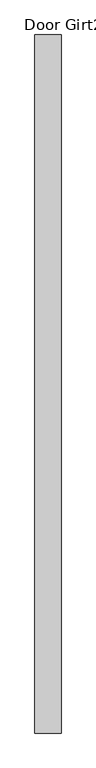
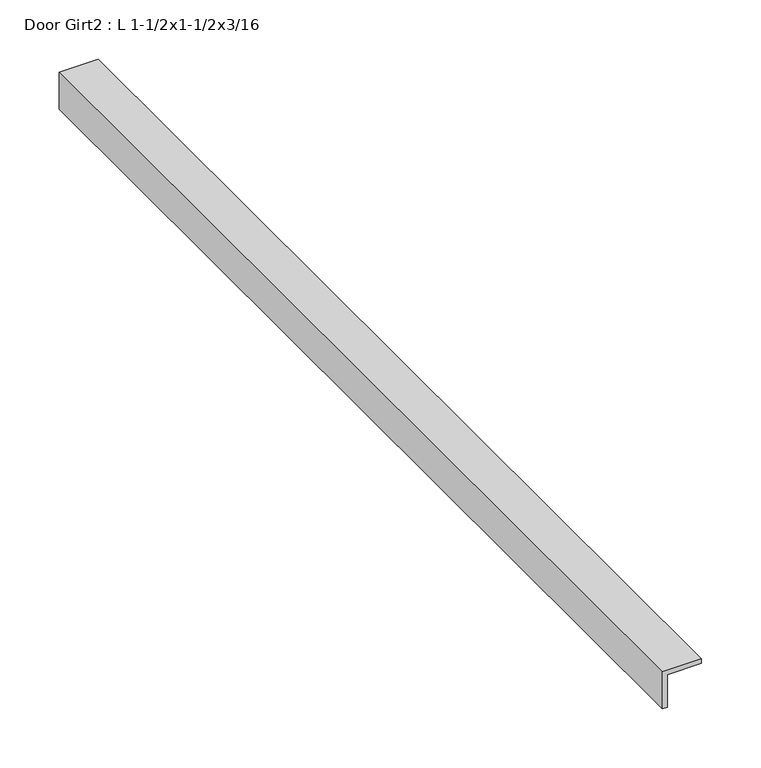
"""IFC4 building model written with IfcOpenShell, lengths in millimetres: proxy geometry, Door Girt2 : L 1-1/2x1-1/2x3/16."""

from ifc_helpers import new_model, si_unit, frame, origin, place, context, project, spatial, polyline, outline, extrude, source, transform, mapped, element, save


def door_girt2_l_1_1_2x1_1_2x3_16_4184d8b8(model_context):
    return source(origin(), model_context, "Body", "SweptSolid", [
        extrude(outline(polyline([(812.8, 587403.9934739), (812.8, 587365.8934739), (774.7, 587365.8934739), (774.7, 587370.6559739), (808.0375, 587370.6559739), (808.0375, 587403.9934739), (812.8, 587403.9934739)])), frame((0.0, -535163.4663841, 0.0), z_axis=(0.0, 1.0, 0.0), x_axis=(0.0, 0.0, 1.0)), (0.0, 0.0, 1.0), 1017.5875),
    ])


if __name__ == "__main__":
    model = new_model("IFC4")
    model_context = context("Model", 3, world=origin())
    ifc_project = project(units=[si_unit("LENGTHUNIT", "METRE", prefix="MILLI")], contexts=[model_context])
    site = spatial("IfcSite", under=ifc_project)
    building = spatial("IfcBuilding", under=site)
    placement = place(None, origin())
    door_girt2_l_1_1_2x1_1_2x3_16_shape = door_girt2_l_1_1_2x1_1_2x3_16_4184d8b8(model_context)
    element("IfcBuildingElementProxy", 1, Name="Door Girt2 : L 1-1/2x1-1/2x3/16", ObjectType="Door Girt2 : L 1-1/2x1-1/2x3/16", at=placement, inside=building, context=model_context, shape_type="MappedRepresentation", body=[
        mapped(door_girt2_l_1_1_2x1_1_2x3_16_shape, transform((0.0, 0.0, 0.0), x_axis=(1.0, 0.0, 0.0), y_axis=(0.0, 1.0, 0.0), z_axis=(0.0, 0.0, 1.0))),
    ])
    save(model, "model.ifc")

# Revit data of these elements
# Element 1 (IfcBuildingElementProxy, "Door Girt2 : L 1-1/2x1-1/2x3/16")
#   Materials on its faces: "1-1/2\"X1-1/2\" GALV. STL L"
# Materials
#   "1-1/2\"X1-1/2\" GALV. STL L": class "Generic", colour RGB 211 211 207, transparency 0, Cost = 0
